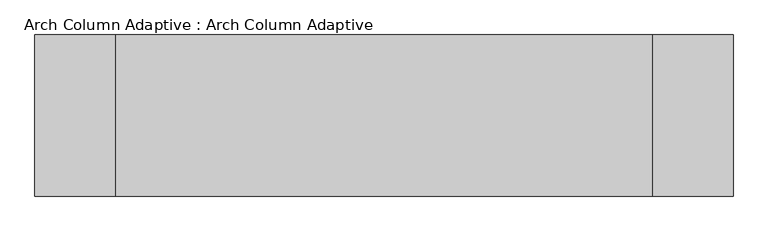
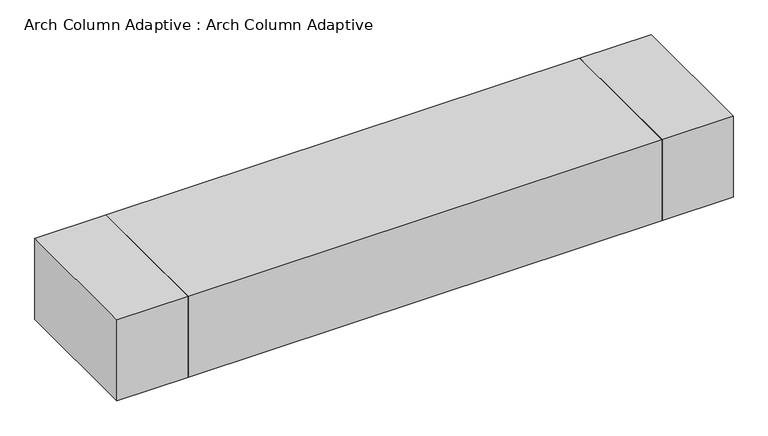
"""IFC4 building model written with IfcOpenShell, lengths in millimetres: proxy geometry, Arch Column Adaptive : Arch Column Adaptive."""

import ifcopenshell
import ifcopenshell.guid

model = None  # the IFC model being written
_history = None  # IfcOwnerHistory: only IFC2X3 demands one
_inside = {}  # id of a spatial element -> (the spatial element, [elements in it])
_under = {}  # id of a project, library or spatial element -> (it, [spatial elements below it])
_declared = {}  # id of a project -> (the project, [libraries it declares])
_typed = {}  # id of a type object -> (the type object, [elements of that type])
_made_of = {}  # id of a material, layer set ... -> (it, [elements and type objects made of it])


def new_model(schema):
    """Start an empty IFC model of exactly this schema.

    Asked for "IFC4X3", IfcOpenShell would pick the latest addendum, in which some entities
    have other attributes; the version numbers below select the first issue.
    IFC2X3 requires an IfcOwnerHistory on every rooted entity: one is made here for all.
    """
    global model, _history
    if schema == "IFC4X3":
        model = ifcopenshell.file(schema_version=(4, 3, 0, 0))
    else:
        model = ifcopenshell.file(schema=schema)
    _inside.clear()
    _under.clear()
    _declared.clear()
    _typed.clear()
    _made_of.clear()
    _history = None
    if model.schema == "IFC2X3":
        org = make("IfcOrganization", Name="unknown")
        user = make(
            "IfcPersonAndOrganization",
            ThePerson=make("IfcPerson", FamilyName="unknown"),
            TheOrganization=org,
        )
        app = make(
            "IfcApplication",
            ApplicationDeveloper=org,
            Version="unknown",
            ApplicationFullName="unknown",
            ApplicationIdentifier="unknown",
        )
        _history = make(
            "IfcOwnerHistory",
            OwningUser=user,
            OwningApplication=app,
            ChangeAction="ADDED",
            CreationDate=0,
        )
    return model


def make(cls, **values):
    """One entity of the class cls with the attributes given. An attribute that is None is left unset."""
    return model.create_entity(
        cls, **{name: value for name, value in values.items() if value is not None}
    )


def rooted(cls, **values):
    """An entity with a GlobalId (a new one), such as an element, a storey or a relation."""
    return make(cls, GlobalId=ifcopenshell.guid.new(), OwnerHistory=_history, **values)


def si_unit(unit_type, name, prefix=None):
    """IfcSIUnit, for example si_unit("LENGTHUNIT", "METRE", prefix="MILLI")."""
    return make("IfcSIUnit", UnitType=unit_type, Prefix=prefix, Name=name)


def assignment(units):
    """IfcUnitAssignment: the units of a project."""
    return None if units is None else make("IfcUnitAssignment", Units=units)


def point(xyz):
    """IfcCartesianPoint."""
    return None if xyz is None else make("IfcCartesianPoint", Coordinates=xyz)


def direction(xyz):
    """IfcDirection."""
    return None if xyz is None else make("IfcDirection", DirectionRatios=xyz)


def frame(location, z_axis=None, x_axis=None):
    """IfcAxis2Placement3D, a coordinate frame: its origin and axes. An axis left out is left unset."""
    return make(
        "IfcAxis2Placement3D",
        Location=point(location),
        Axis=direction(z_axis),
        RefDirection=direction(x_axis),
    )


def origin():
    """The frame at (0, 0, 0) with its axes left unset."""
    return frame((0.0, 0.0, 0.0))


def place(relative_to, where):
    """IfcLocalPlacement: puts the frame where relative to a parent placement (None: the world)."""
    return make(
        "IfcLocalPlacement", PlacementRelTo=relative_to, RelativePlacement=where
    )


def context(
    kind, dimensions, precision=None, world=None, true_north=None, identifier=None
):
    """IfcGeometricRepresentationContext, for example the 3D "Model" context."""
    return make(
        "IfcGeometricRepresentationContext",
        ContextIdentifier=identifier,
        ContextType=kind,
        CoordinateSpaceDimension=dimensions,
        Precision=precision,
        WorldCoordinateSystem=world,
        TrueNorth=true_north,
    )


def project(units=None, contexts=None):
    """IfcProject with its units and contexts."""
    return rooted(
        "IfcProject",
        Name="project",
        RepresentationContexts=contexts,
        UnitsInContext=assignment(units),
    )


def spatial(cls, under=None, at=None, **own):
    """A site, building, storey or space (cls), placed at a placement, below another one or the project."""
    s = rooted(cls, ObjectPlacement=at, **own)
    if under is not None:
        _under.setdefault(under.id(), (under, []))[1].append(s)
    return s


def polyline(points):
    """IfcPolyline through the points."""
    return make("IfcPolyline", Points=[point(p) for p in points])


def outline(outer, holes=None, kind="AREA"):
    """IfcArbitraryClosedProfileDef: a profile drawn as a closed curve; with holes, ...WithVoids."""
    if holes is None:
        return make("IfcArbitraryClosedProfileDef", ProfileType=kind, OuterCurve=outer)
    return make(
        "IfcArbitraryProfileDefWithVoids",
        ProfileType=kind,
        OuterCurve=outer,
        InnerCurves=holes,
    )


def extrude(swept, where, along, depth):
    """IfcExtrudedAreaSolid: the profile swept, set in the frame where, extruded along a direction by depth."""
    return make(
        "IfcExtrudedAreaSolid",
        SweptArea=swept,
        Position=where,
        ExtrudedDirection=direction(along),
        Depth=depth,
    )


def shape(context_of_items, identifier, shape_type, items):
    """IfcShapeRepresentation: the items that make up one representation, for example the "Body"."""
    return make(
        "IfcShapeRepresentation",
        ContextOfItems=context_of_items,
        RepresentationIdentifier=identifier,
        RepresentationType=shape_type,
        Items=items,
    )


def source(mapping_origin, context_of_items, identifier, shape_type, items):
    """IfcRepresentationMap: a shape defined once, which mapped items show again and again."""
    return make(
        "IfcRepresentationMap",
        MappingOrigin=mapping_origin,
        MappedRepresentation=shape(context_of_items, identifier, shape_type, items),
    )


def transform(
    local_origin,
    x_axis=None,
    y_axis=None,
    z_axis=None,
    scale=None,
    scale2=None,
    scale3=None,
    uniform=True,
):
    """IfcCartesianTransformationOperator3D, or its non-uniform kind. x_axis, y_axis, z_axis: its Axis1, 2, 3."""
    if uniform:
        return make(
            "IfcCartesianTransformationOperator3D",
            Axis1=direction(x_axis),
            Axis2=direction(y_axis),
            LocalOrigin=point(local_origin),
            Scale=scale,
            Axis3=direction(z_axis),
        )
    return make(
        "IfcCartesianTransformationOperator3DnonUniform",
        Axis1=direction(x_axis),
        Axis2=direction(y_axis),
        LocalOrigin=point(local_origin),
        Scale=scale,
        Axis3=direction(z_axis),
        Scale2=scale2,
        Scale3=scale3,
    )


def mapped(mapping_source, mapping_target):
    """IfcMappedItem: shows the shape of a source again, moved by a transform."""
    return make(
        "IfcMappedItem", MappingSource=mapping_source, MappingTarget=mapping_target
    )


def made_of(thing, what):
    """Note that an element or type object is made of a material, layer set ...; save() writes the relation."""
    if what is not None:
        _made_of.setdefault(what.id(), (what, []))[1].append(thing)
    return thing


def element(
    cls,
    number,
    at=None,
    inside=None,
    cuts=None,
    type_object=None,
    material=None,
    context=None,
    identifier="Body",
    shape_type=None,
    held_by="IfcProductDefinitionShape",
    body=None,
    shapes=None,
    **own,
):
    """One element of the class cls, such as IfcWall. Its Tag is "e" and its number.

    at: its placement. inside: the storey or other place that contains it. cuts: it is an
    opening in that element (IfcRelVoidsElement). A single representation is given by context,
    identifier, shape_type and body (its items); several are given by shapes. held_by: the class
    of the entity that holds the representations. save() writes the other relations.
    """
    e = rooted(cls, Tag="e%d" % number, ObjectPlacement=at, **own)
    if body is not None:
        shapes = [shape(context, identifier, shape_type, body)]
    if shapes is not None:
        e.Representation = make(held_by, Representations=shapes)
    if inside is not None:
        _inside.setdefault(inside.id(), (inside, []))[1].append(e)
    if cuts is not None:
        rooted(
            "IfcRelVoidsElement", RelatingBuildingElement=cuts, RelatedOpeningElement=e
        )
    if type_object is not None:
        _typed.setdefault(type_object.id(), (type_object, []))[1].append(e)
    return made_of(e, material)


def aggregate(whole, parts):
    """IfcRelAggregates: a whole, such as a stair, and the parts it consists of."""
    return rooted("IfcRelAggregates", RelatingObject=whole, RelatedObjects=parts)


def save(model, path):
    """Write the relations noted so far, then the file.

    IfcRelAggregates (storeys below a building ...), IfcRelContainedInSpatialStructure (elements
    in a storey), IfcRelDefinesByType, IfcRelAssociatesMaterial and IfcRelDeclares: one each for
    every whole, place, type object, material and project.
    """
    for whole, parts in _under.values():
        aggregate(whole, parts)
    for where, things in _inside.values():
        rooted(
            "IfcRelContainedInSpatialStructure",
            RelatedElements=things,
            RelatingStructure=where,
        )
    for kind, things in _typed.values():
        rooted("IfcRelDefinesByType", RelatedObjects=things, RelatingType=kind)
    for what, things in _made_of.values():
        rooted("IfcRelAssociatesMaterial", RelatedObjects=things, RelatingMaterial=what)
    for by, libraries in _declared.values():
        rooted("IfcRelDeclares", RelatingContext=by, RelatedDefinitions=libraries)
    model.write(path)


def arch_column_adaptive_arch_column_adaptive_cbfe978d(model_context):
    return source(origin(), model_context, "Body", "SweptSolid", [
        extrude(outline(polyline([(5000.0, -1500.0), (5000.0, 1500.0), (6500.0, 1500.0), (6500.0, -1500.0), (5000.0, -1500.0)])), frame((0.0, 0.0, 51255.6), z_axis=(0.0, 0.0, 1.0), x_axis=(1.0, 0.0, 0.0)), (0.0, 0.0, 1.0), 1800.0),
        extrude(outline(polyline([(-5000.0, 1500.0), (-5000.0, -1500.0), (-6500.0, -1500.0), (-6500.0, 1500.0), (-5000.0, 1500.0)])), frame((0.0, 0.0, 51255.6), z_axis=(0.0, 0.0, 1.0), x_axis=(1.0, 0.0, 0.0)), (0.0, 0.0, 1.0), 1800.0),
        extrude(outline(polyline([(-5000.0, -1500.0), (-5000.0, 1500.0), (5000.0, 1500.0), (5000.0, -1500.0), (-5000.0, -1500.0)])), frame((0.0, 0.0, 51255.6), z_axis=(0.0, 0.0, 1.0), x_axis=(1.0, 0.0, 0.0)), (0.0, 0.0, 1.0), 1800.0),
    ])


if __name__ == "__main__":
    model = new_model("IFC4")
    model_context = context("Model", 3, world=origin())
    ifc_project = project(units=[si_unit("LENGTHUNIT", "METRE", prefix="MILLI")], contexts=[model_context])
    site = spatial("IfcSite", under=ifc_project)
    building = spatial("IfcBuilding", under=site)
    placement = place(None, origin())
    arch_column_adaptive_arch_column_adaptive_shape = arch_column_adaptive_arch_column_adaptive_cbfe978d(model_context)
    element("IfcBuildingElementProxy", 1, Name="Arch Column Adaptive : Arch Column Adaptive", ObjectType="Arch Column Adaptive : Arch Column Adaptive", at=placement, inside=building, context=model_context, shape_type="MappedRepresentation", body=[
        mapped(arch_column_adaptive_arch_column_adaptive_shape, transform((0.0, 0.0, 0.0), x_axis=(1.0, 0.0, 0.0), y_axis=(0.0, 1.0, 0.0), z_axis=(0.0, 0.0, 1.0))),
    ])
    save(model, "model.ifc")

# Revit data of these elements
# Type "Arch Column Adaptive : Arch Column Adaptive"
#   Top Width = 3000 mm
#   Length [instance default] = 21000 mm
#   Height [instance default] = 50000 mm
#   Default Elevation = 0
# Element 1 (IfcBuildingElementProxy, "Arch Column Adaptive : Arch Column Adaptive")
#   Height = 51255.6 mm
